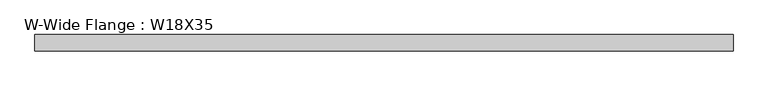
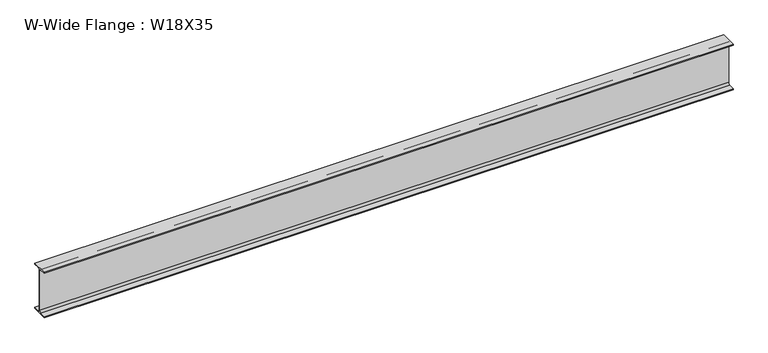
"""IFC4 building model written with IfcOpenShell, lengths in millimetres: beam geometry, W-Wide Flange : W18X35."""

from ifc_helpers import new_model, si_unit, point, frame, frame_2d, origin, place, context, project, spatial, polyline, circle_curve, trimmed, segment, composite_curve, outline, extrude, source, transform, mapped, element, save


def w_wide_flange_w18x35_15e55470(model_context):
    return source(origin(), model_context, "Body", "SweptSolid", [
        extrude(outline(composite_curve([segment(polyline([(-76.2, -213.995), (-21.59, -213.995)]), True, "CONTINUOUS"), segment(trimmed(circle_curve(frame_2d((-21.59, -196.215)), 17.78), [point((-21.59, -213.995))], [point((-3.81, -196.215))], True, "CARTESIAN"), True, "CONTINUOUS"), segment(polyline([(-3.81, -196.215), (-3.81, 196.215)]), True, "CONTINUOUS"), segment(trimmed(circle_curve(frame_2d((-21.59, 196.215)), 17.78), [point((-3.81, 196.215))], [point((-21.59, 213.995))], True, "CARTESIAN"), True, "CONTINUOUS"), segment(polyline([(-21.59, 213.995), (-76.2, 213.995), (-76.2, 224.79), (76.2, 224.79), (76.2, 213.995), (21.59, 213.995)]), True, "CONTINUOUS"), segment(trimmed(circle_curve(frame_2d((21.59, 196.215)), 17.78), [point((21.59, 213.995))], [point((3.81, 196.215))], True, "CARTESIAN"), True, "CONTINUOUS"), segment(polyline([(3.81, 196.215), (3.81, -196.215)]), True, "CONTINUOUS"), segment(trimmed(circle_curve(frame_2d((21.59, -196.215)), 17.78), [point((3.81, -196.215))], [point((21.59, -213.995))], True, "CARTESIAN"), True, "CONTINUOUS"), segment(polyline([(21.59, -213.995), (76.2, -213.995), (76.2, -224.79), (-76.2, -224.79), (-76.2, -213.995)]), True, "CONTINUOUS")], self_intersect=False)), frame((-3270.25, 0.0, 0.0), z_axis=(1.0, 0.0, 0.0), x_axis=(0.0, 1.0, 0.0)), (0.0, 0.0, 1.0), 6443.98),
    ])


if __name__ == "__main__":
    model = new_model("IFC4")
    model_context = context("Model", 3, world=origin())
    ifc_project = project(units=[si_unit("LENGTHUNIT", "METRE", prefix="MILLI")], contexts=[model_context])
    site = spatial("IfcSite", under=ifc_project)
    building = spatial("IfcBuilding", under=site)
    placement = place(None, origin())
    w_wide_flange_w18x35_shape = w_wide_flange_w18x35_15e55470(model_context)
    element("IfcBeam", 1, ObjectType="W-Wide Flange : W18X35", at=placement, inside=building, context=model_context, shape_type="MappedRepresentation", body=[
        mapped(w_wide_flange_w18x35_shape, transform((0.0, 0.0, 0.0), x_axis=(1.0, 0.0, 0.0), y_axis=(0.0, 1.0, 0.0), z_axis=(0.0, 0.0, 1.0))),
    ])
    save(model, "model.ifc")

# Revit data of these elements
# Type "W-Wide Flange : W18X35"
#   Assembly Code = "B10"
#   W = 35
#   Start Extension Calculation [instance default] = 10' - 0"
#   Start Extension [instance default] = -0' - 0 1/2"
#   End Extension Calculation [instance default] = 10' - 0"
#   End Extension [instance default] = -0' - 0 1/2"
#   Length [instance default] = 5' - 0"
#   bf = 0' - 6"
#   d = 1' - 5.7"
#   k = 0' - 1 1/8"
#   k2 = 0' - 0.7"
#   tf = 0' - 0.425"
#   tw = 0' - 0.3"
#   A = 0.0715278 SF
#   Beam Material [instance default] = Metal - Steel - ASTM A992
# Element 1 (IfcBeam, "W-Wide Flange : W18X35")
#   Materials on its faces: "Metal - Steel - ASTM A992"
# Materials
#   "Metal - Steel - ASTM A992": class "Metal", colour RGB 128 0 0, transparency 0
